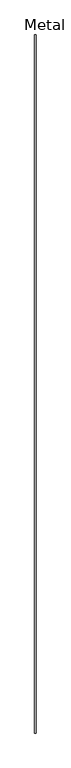
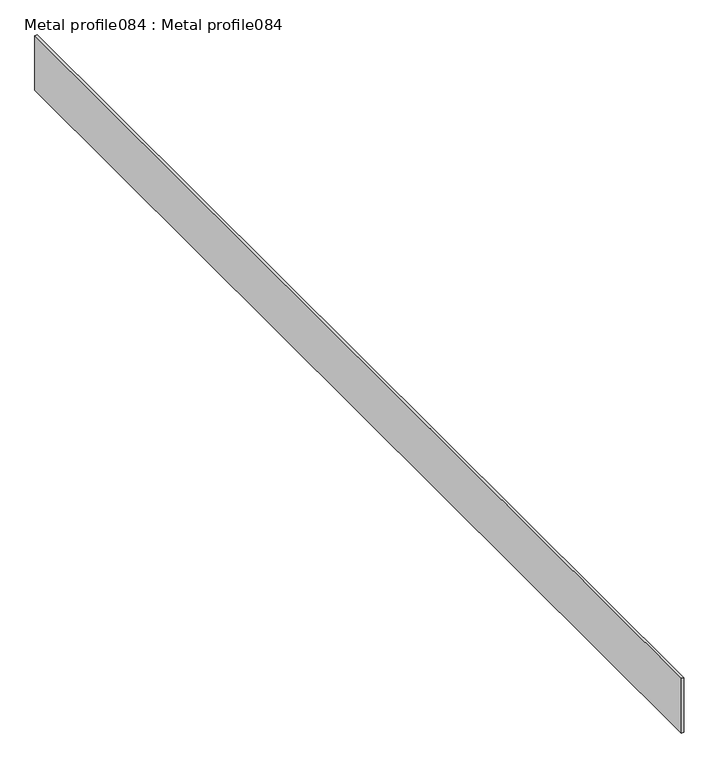
"""IFC4 building model written with IfcOpenShell, lengths in millimetres: proxy geometry, Metal profile084 : Metal profile084."""

from ifc_helpers import new_model, si_unit, frame, origin, place, context, project, spatial, polyline, outline, extrude, source, transform, mapped, element, save


def metal_profile084_metal_profile084_53555982(model_context):
    return source(origin(), model_context, "Body", "SweptSolid", [
        extrude(outline(polyline([(-7053.5948688, 7982.1531721), (-7057.5948688, 7982.1531721), (-7057.5948688, 9982.1531721), (-7053.5948688, 9982.1531721), (-7053.5948688, 7982.1531721)])), frame((0.0, 0.0, 40157.4057921), z_axis=(0.0, 0.0, 1.0), x_axis=(1.0, 0.0, 0.0)), (0.0, 0.0, 1.0), 103.0664062),
    ])


if __name__ == "__main__":
    model = new_model("IFC4")
    model_context = context("Model", 3, world=origin())
    ifc_project = project(units=[si_unit("LENGTHUNIT", "METRE", prefix="MILLI")], contexts=[model_context])
    site = spatial("IfcSite", under=ifc_project)
    building = spatial("IfcBuilding", under=site)
    placement = place(None, origin())
    metal_profile084_metal_profile084_shape = metal_profile084_metal_profile084_53555982(model_context)
    element("IfcBuildingElementProxy", 1, Name="Metal profile084 : Metal profile084", ObjectType="Metal profile084 : Metal profile084", at=placement, inside=building, context=model_context, shape_type="MappedRepresentation", body=[
        mapped(metal_profile084_metal_profile084_shape, transform((0.0, 0.0, 0.0), x_axis=(1.0, 0.0, 0.0), y_axis=(0.0, 1.0, 0.0), z_axis=(0.0, 0.0, 1.0))),
    ])
    save(model, "model.ifc")

# Revit data of these elements
# Type "Metal profile084 : Metal profile084"
#   NameOverride = "Metal profile084"
# Element 1 (IfcBuildingElementProxy, "Metal profile084 : Metal profile084")
#   Materials on its faces: "FIXATION SYSTEM FOR GLASS RAILING AS NEEDED"
# Materials
#   "FIXATION SYSTEM FOR GLASS RAILING AS NEEDED": class "Unassigned", colour RGB 128 128 128, transparency 0
